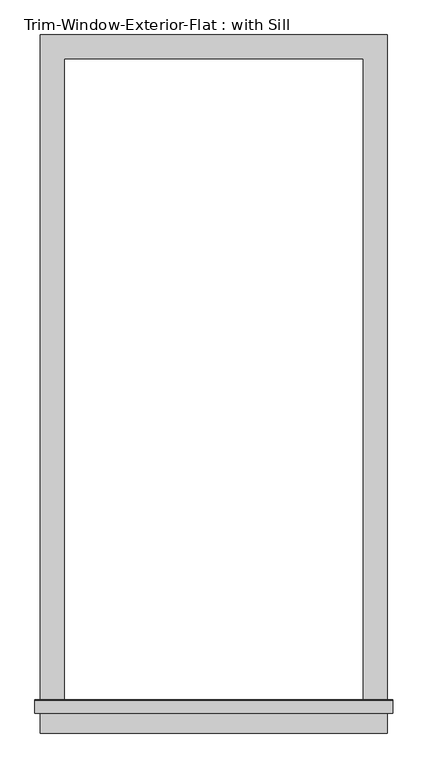
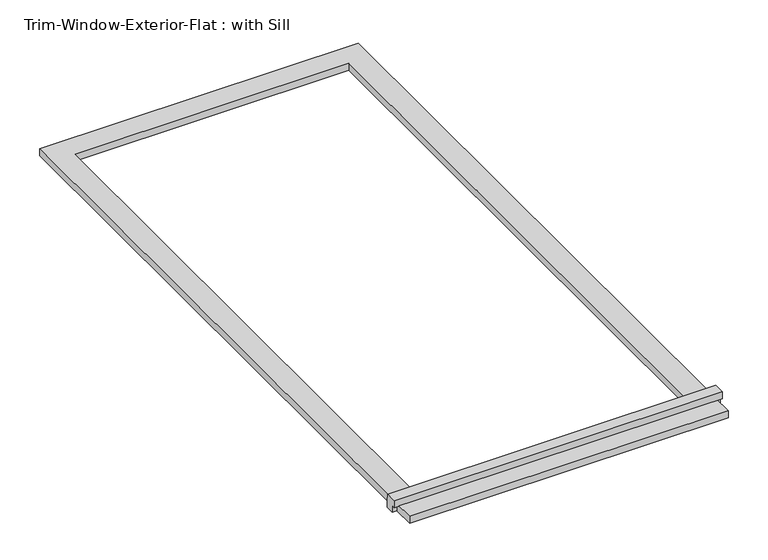
"""IFC4 building model written with IfcOpenShell, lengths in millimetres: proxy geometry, Trim-Window-Exterior-Flat : with Sill."""

from ifc_helpers import new_model, si_unit, frame, origin, origin_with_axes, place, context, project, spatial, polyline, outline, extrude, source, transform, mapped, element, save


def trim_window_exterior_flat_with_sill_ca40e5bd(model_context):
    return source(origin(), model_context, "Body", "SweptSolid", [
        extrude(outline(polyline([(412.75, -1546.1823709), (412.75, -1603.3323709), (-412.75, -1603.3323709), (-412.75, -1546.1823709), (412.75, -1546.1823709)])), origin_with_axes(), (0.0, 0.0, 1.0), 19.05),
        extrude(outline(polyline([(-1555.75, 38.1), (-1526.4580645, 38.1), (-1524.0, 19.05), (-1524.0, 0.0), (-1546.1823709, 0.0), (-1546.1823709, 19.05), (-1555.75, 19.05), (-1555.75, 38.1)])), frame((-425.45, 0.0, 0.0), z_axis=(1.0, 0.0, 0.0), x_axis=(0.0, 1.0, 0.0)), (0.0, 0.0, 1.0), 850.9),
        extrude(outline(polyline([(-412.75, 57.15), (412.75, 57.15), (412.75, -1524.0), (355.6, -1524.0), (355.6, 0.0), (-355.6, 0.0), (-355.6, -1524.0), (-412.75, -1524.0), (-412.75, 57.15)])), origin_with_axes(), (0.0, 0.0, 1.0), 19.05),
    ])


if __name__ == "__main__":
    model = new_model("IFC4")
    model_context = context("Model", 3, world=origin())
    ifc_project = project(units=[si_unit("LENGTHUNIT", "METRE", prefix="MILLI")], contexts=[model_context])
    site = spatial("IfcSite", under=ifc_project)
    building = spatial("IfcBuilding", under=site)
    placement = place(None, origin())
    trim_window_exterior_flat_with_sill_shape = trim_window_exterior_flat_with_sill_ca40e5bd(model_context)
    element("IfcBuildingElementProxy", 1, Name="Trim-Window-Exterior-Flat : with Sill", ObjectType="Trim-Window-Exterior-Flat : with Sill", at=placement, inside=building, context=model_context, shape_type="MappedRepresentation", body=[
        mapped(trim_window_exterior_flat_with_sill_shape, transform((0.0, 0.0, 0.0), x_axis=(1.0, 0.0, 0.0), y_axis=(0.0, 1.0, 0.0), z_axis=(0.0, 0.0, 1.0))),
    ])
    save(model, "model.ifc")

# Revit data of these elements
# Type "Trim-Window-Exterior-Flat : with Sill"
#   Trim Width = 0' - 2 1/4"
#   Trim Thickness_Picture Frame = 0' - 1 1/4"
#   Trim Thickness_with Sill = 0' - 0 3/4"
#   Sill Thickness = 0' - 1 1/4"
#   Opening Width [instance default] = 2' - 0"
#   Opening Height [instance default] = 3' - 0"
#   Default Elevation = 4' - 0"
#   Sill = yes
#   Picture Frame = no
#   Trim Material [instance default] = none
# Element 1 (IfcBuildingElementProxy, "Trim-Window-Exterior-Flat : with Sill")
#   Opening Width = 2' - 4"
#   Opening Height = 5' - 0"
#   Trim Material = Clad - White
#   Materials on its faces: "Clad - White"
# Materials
#   "Clad - White": class "Wood", colour RGB 242 242 238, transparency 0, Cost = 0
